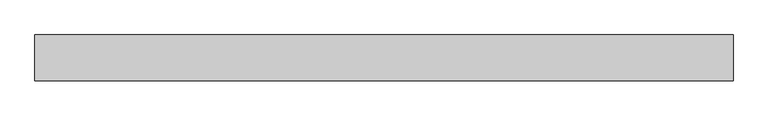
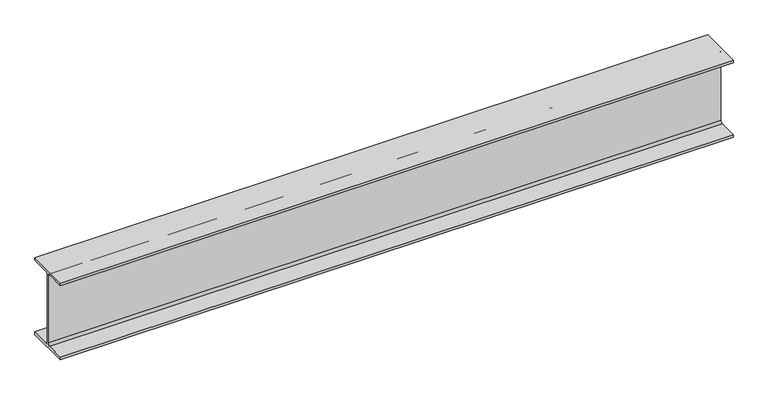
"""IFC4 building model written with IfcOpenShell, lengths in millimetres: beam geometry, Old_Steel Beam_H-KSD3502 : H_SB_ASB_H-250×125x6x9."""

from ifc_helpers import new_model, si_unit, point, frame, frame_2d, origin, place, context, project, spatial, polyline, circle_curve, trimmed, segment, composite_curve, outline, extrude, source, transform, mapped, element, save


def beam_9f3c0b06(model_context):
    return source(origin(), model_context, "Body", "SweptSolid", [
        extrude(outline(composite_curve([segment(polyline([(82.5, -141.5), (82.5, -151.7), (-82.5, -151.7), (-82.5, -141.5), (-11.9, -141.5)]), True, "CONTINUOUS"), segment(trimmed(circle_curve(frame_2d((-11.9, -132.6)), 8.9), [point((-11.9, -141.5))], [point((-3.0, -132.6))], True, "CARTESIAN"), True, "CONTINUOUS"), segment(polyline([(-3.0, -132.6), (-3.0, 132.6)]), True, "CONTINUOUS"), segment(trimmed(circle_curve(frame_2d((-11.9, 132.6)), 8.9), [point((-3.0, 132.6))], [point((-11.9, 141.5))], True, "CARTESIAN"), True, "CONTINUOUS"), segment(polyline([(-11.9, 141.5), (-82.5, 141.5), (-82.5, 151.7), (82.5, 151.7), (82.5, 141.5), (11.9, 141.5)]), True, "CONTINUOUS"), segment(trimmed(circle_curve(frame_2d((11.9, 132.6)), 8.9), [point((11.9, 141.5))], [point((3.0, 132.6))], True, "CARTESIAN"), True, "CONTINUOUS"), segment(polyline([(3.0, 132.6), (3.0, -132.6)]), True, "CONTINUOUS"), segment(trimmed(circle_curve(frame_2d((11.9, -132.6)), 8.9), [point((3.0, -132.6))], [point((11.9, -141.5))], True, "CARTESIAN"), True, "CONTINUOUS"), segment(polyline([(11.9, -141.5), (82.5, -141.5)]), True, "CONTINUOUS")], self_intersect=False)), frame((-1337.3, 0.0, 0.0), z_axis=(1.0, 0.0, 0.0), x_axis=(0.0, 1.0, 0.0)), (0.0, 0.0, 1.0), 2511.6),
    ])


if __name__ == "__main__":
    model = new_model("IFC4")
    model_context = context("Model", 3, world=origin())
    ifc_project = project(units=[si_unit("LENGTHUNIT", "METRE", prefix="MILLI")], contexts=[model_context])
    site = spatial("IfcSite", under=ifc_project)
    building = spatial("IfcBuilding", under=site)
    placement = place(None, origin())
    beam_shape = beam_9f3c0b06(model_context)
    element("IfcBeam", 1, ObjectType="Old_Steel Beam_H-KSD3502 : H_SB_ASB_H-250×125x6x9", at=placement, inside=building, context=model_context, shape_type="MappedRepresentation", body=[
        mapped(beam_shape, transform((0.0, 0.0, 0.0), x_axis=(1.0, 0.0, 0.0), y_axis=(0.0, 1.0, 0.0), z_axis=(0.0, 0.0, 1.0))),
    ])
    save(model, "model.ifc")

# Revit data of these elements
# Type "Old_Steel Beam_H-KSD3502 : H_SB_ASB_H-250×125x6x9"
#   Width = 12.5 cm
#   Web Thickness = 0.6 cm
#   Web Fillet = 1.2 cm
#   Warping Constant = 42539.8 cm⁶
#   Torsional Moment of Inertia = 7.8102 cm⁴
#   Torsional Modulus = 1.0 cm³
#   Section Area = 37.66 cm²
#   Plastic Modulus weak axis = 73.1 cm³
#   Plastic Modulus strong axis = 366.0 cm³
#   Perimeter = 0.97 m²/m
#   Nominal Weight = 29.60 kgf/m
#   Moment of Inertia weak axis = 294.00 cm⁴
#   Moment of Inertia strong axis = 4050.00 cm⁴
#   Height = 25.0 cm
#   Flange Thickness = 0.9 cm
#   Elastic Modulus weak axis = 47.0 cm³
#   Elastic Modulus strong axis = 324.0 cm³
#   Centroid Vertical = 12.5 cm
#   Centroid Horizontal = 6.25 cm
#   Length [instance default] = 1.5240 m
#   Structural Material [instance default] = Steel, 45-345
#   Assembly Code = ""
# Element 1 (IfcBeam, "Old_Steel Beam_H-KSD3502 : H_SB_ASB_H-250×125x6x9")
#   Structural Material = none
# Materials
#   "Steel, 45-345": class "Metal", colour RGB 189 187 185, transparency 0, Description = "Steel 345 MPa", Cost = 0
